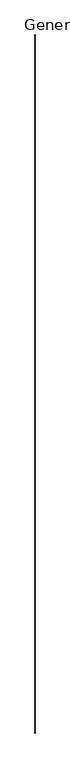
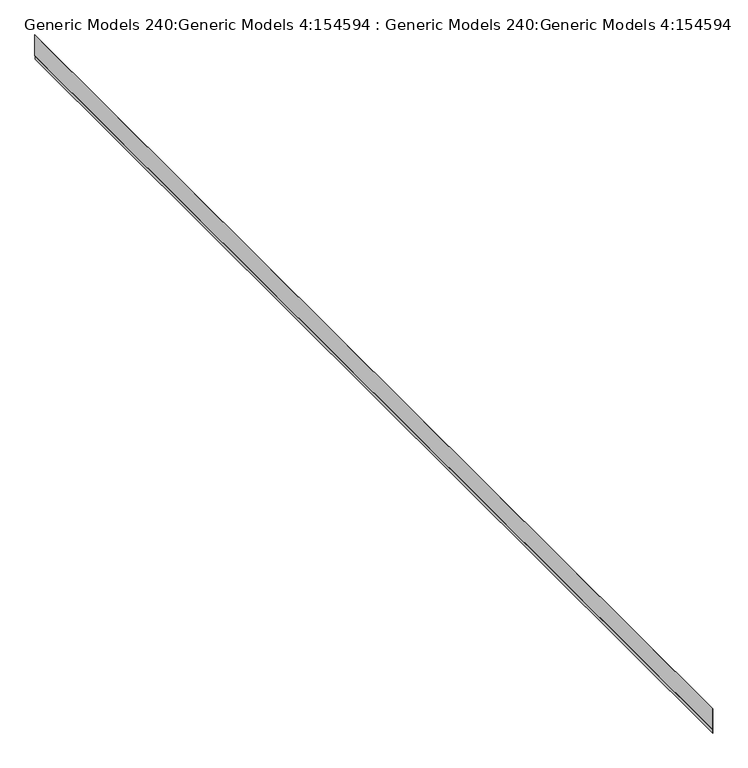
"""IFC4 building model written with IfcOpenShell, lengths in millimetres: proxy geometry, Generic Models 240:Generic Models 4:154594 : Generic Models 240:Generic Models 4:154594."""

from ifc_helpers import new_model, si_unit, frame, origin, place, context, project, spatial, polyline, outline, extrude, source, transform, mapped, element, save


def generic_models_240_generic_models_4_154594_generic_models_8d005530(model_context):
    return source(origin(), model_context, "Body", "SweptSolid", [
        extrude(outline(polyline([(3366.142086, 1597.6373761), (3013.7444211, 1597.6373761), (3008.1027003, 1599.6907945), (2960.535851, 1599.6907945), (2960.535851, 1600.4845445), (3008.2426599, 1600.4845445), (3013.8843806, 1598.4311261), (3366.142086, 1598.4311261), (3366.142086, 1597.6373761)])), frame((0.0, -8838.4871142, 0.0), z_axis=(0.0, 1.0, 0.0), x_axis=(0.0, 0.0, 1.0)), (0.0, 0.0, 1.0), 18643.6),
    ])


if __name__ == "__main__":
    model = new_model("IFC4")
    model_context = context("Model", 3, world=origin())
    ifc_project = project(units=[si_unit("LENGTHUNIT", "METRE", prefix="MILLI")], contexts=[model_context])
    site = spatial("IfcSite", under=ifc_project)
    building = spatial("IfcBuilding", under=site)
    placement = place(None, origin())
    generic_models_240_generic_models_4_154594_generic_models_shape = generic_models_240_generic_models_4_154594_generic_models_8d005530(model_context)
    element("IfcBuildingElementProxy", 1, Name="Generic Models 240:Generic Models 4:154594 : Generic Models 240:Generic Models 4:154594", ObjectType="Generic Models 240:Generic Models 4:154594 : Generic Models 240:Generic Models 4:154594", at=placement, inside=building, context=model_context, shape_type="MappedRepresentation", body=[
        mapped(generic_models_240_generic_models_4_154594_generic_models_shape, transform((0.0, 0.0, 0.0), x_axis=(1.0, 0.0, 0.0), y_axis=(0.0, 1.0, 0.0), z_axis=(0.0, 0.0, 1.0))),
    ])
    save(model, "model.ifc")

# Revit data of these elements
# Type "Generic Models 240:Generic Models 4:154594 : Generic Models 240:Generic Models 4:154594"
#   NameOverride = "Generic Models 240:Generic Models 4:154594"
#   ObjectTypeOverride = "Generic Models 240:Generic Models 4"
#   Reference = "Generic Models 4"
#   Category = "Generic Models"
#   Tag = "154594"
# Element 1 (IfcBuildingElementProxy, "Generic Models 240:Generic Models 4:154594 : Generic Models 240:Generic Models 4:154594")
#   Materials on its faces: "_DRAINABLE BUILDING WRAP 24696"
# Materials
#   "_DRAINABLE BUILDING WRAP 24696": class "Unassigned", colour RGB 67 154 161, transparency 0
